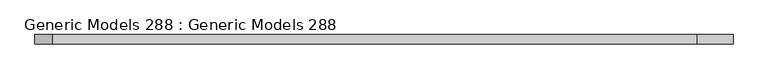
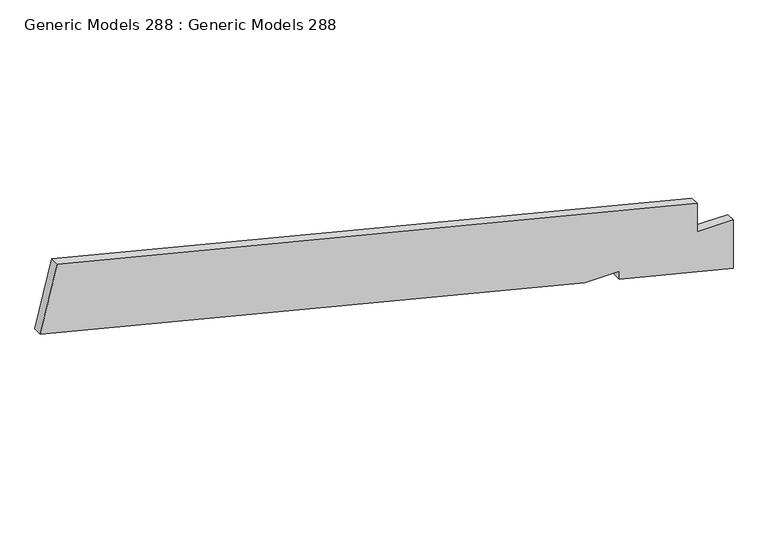
"""IFC4 building model written with IfcOpenShell, lengths in millimetres: proxy geometry, Generic Models 288 : Generic Models 288."""

from ifc_helpers import new_model, si_unit, frame, origin, place, context, project, spatial, polyline, outline, extrude, source, transform, mapped, element, save


def generic_models_288_generic_models_288_55758940(model_context):
    return source(origin(), model_context, "Body", "SweptSolid", [
        extrude(outline(polyline([(129696.0771811, 1936.5763704), (130347.4874812, -669.06483), (130070.2692618, -738.3693849), (129515.8328229, 1479.3763704), (129515.8328229, 1619.0763704), (129480.9078229, 1619.0763704), (129365.0203229, 2082.6263704), (129573.98733, 2082.6263704), (129573.98733, 1936.5763704), (129696.0771811, 1936.5763704)])), frame((0.0, 5408.0122548, 0.0), z_axis=(0.0, 1.0, 0.0), x_axis=(0.0, 0.0, 1.0)), (0.0, 0.0, 1.0), 38.1),
    ])


if __name__ == "__main__":
    model = new_model("IFC4")
    model_context = context("Model", 3, world=origin())
    ifc_project = project(units=[si_unit("LENGTHUNIT", "METRE", prefix="MILLI")], contexts=[model_context])
    site = spatial("IfcSite", under=ifc_project)
    building = spatial("IfcBuilding", under=site)
    placement = place(None, origin())
    generic_models_288_generic_models_288_shape = generic_models_288_generic_models_288_55758940(model_context)
    element("IfcBuildingElementProxy", 1, Name="Generic Models 288 : Generic Models 288", ObjectType="Generic Models 288 : Generic Models 288", at=placement, inside=building, context=model_context, shape_type="MappedRepresentation", body=[
        mapped(generic_models_288_generic_models_288_shape, transform((0.0, 0.0, 0.0), x_axis=(1.0, 0.0, 0.0), y_axis=(0.0, 1.0, 0.0), z_axis=(0.0, 0.0, 1.0))),
    ])
    save(model, "model.ifc")

# Revit data of these elements
# Element 1 (IfcBuildingElementProxy, "Generic Models 288 : Generic Models 288")
#   Materials on its faces: "_STRUCTURAL MEMBER (SEE STRUCT. DWGS)"
# Materials
#   "_STRUCTURAL MEMBER (SEE STRUCT. DWGS)": class "Generic", colour RGB 209 182 141, transparency 0, Cost = 0
